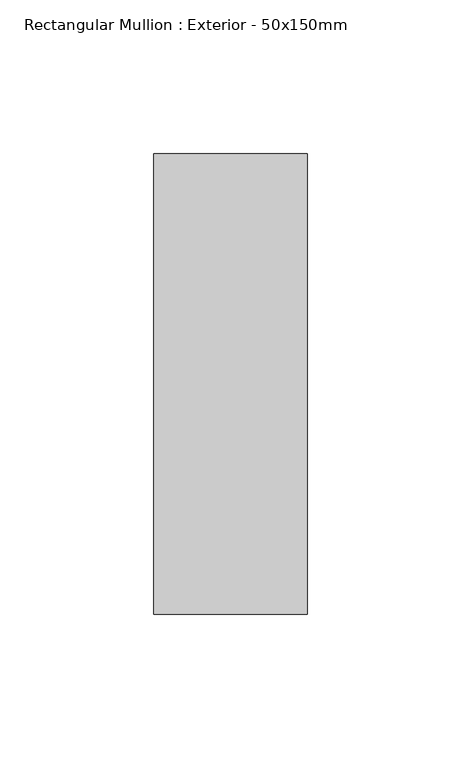
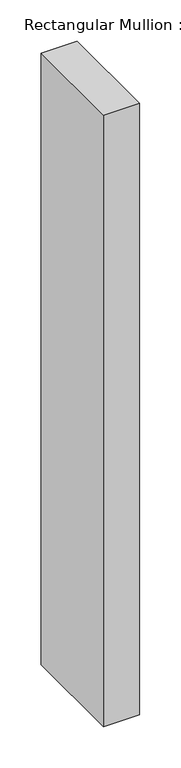
"""IFC4 building model written with IfcOpenShell, lengths in millimetres: member geometry, Rectangular Mullion : Exterior - 50x150mm."""

import ifcopenshell
import ifcopenshell.guid

model = None  # the IFC model being written
_history = None  # IfcOwnerHistory: only IFC2X3 demands one
_inside = {}  # id of a spatial element -> (the spatial element, [elements in it])
_under = {}  # id of a project, library or spatial element -> (it, [spatial elements below it])
_declared = {}  # id of a project -> (the project, [libraries it declares])
_typed = {}  # id of a type object -> (the type object, [elements of that type])
_made_of = {}  # id of a material, layer set ... -> (it, [elements and type objects made of it])


def new_model(schema):
    """Start an empty IFC model of exactly this schema.

    Asked for "IFC4X3", IfcOpenShell would pick the latest addendum, in which some entities
    have other attributes; the version numbers below select the first issue.
    IFC2X3 requires an IfcOwnerHistory on every rooted entity: one is made here for all.
    """
    global model, _history
    if schema == "IFC4X3":
        model = ifcopenshell.file(schema_version=(4, 3, 0, 0))
    else:
        model = ifcopenshell.file(schema=schema)
    _inside.clear()
    _under.clear()
    _declared.clear()
    _typed.clear()
    _made_of.clear()
    _history = None
    if model.schema == "IFC2X3":
        org = make("IfcOrganization", Name="unknown")
        user = make(
            "IfcPersonAndOrganization",
            ThePerson=make("IfcPerson", FamilyName="unknown"),
            TheOrganization=org,
        )
        app = make(
            "IfcApplication",
            ApplicationDeveloper=org,
            Version="unknown",
            ApplicationFullName="unknown",
            ApplicationIdentifier="unknown",
        )
        _history = make(
            "IfcOwnerHistory",
            OwningUser=user,
            OwningApplication=app,
            ChangeAction="ADDED",
            CreationDate=0,
        )
    return model


def make(cls, **values):
    """One entity of the class cls with the attributes given. An attribute that is None is left unset."""
    return model.create_entity(
        cls, **{name: value for name, value in values.items() if value is not None}
    )


def rooted(cls, **values):
    """An entity with a GlobalId (a new one), such as an element, a storey or a relation."""
    return make(cls, GlobalId=ifcopenshell.guid.new(), OwnerHistory=_history, **values)


def si_unit(unit_type, name, prefix=None):
    """IfcSIUnit, for example si_unit("LENGTHUNIT", "METRE", prefix="MILLI")."""
    return make("IfcSIUnit", UnitType=unit_type, Prefix=prefix, Name=name)


def assignment(units):
    """IfcUnitAssignment: the units of a project."""
    return None if units is None else make("IfcUnitAssignment", Units=units)


def point(xyz):
    """IfcCartesianPoint."""
    return None if xyz is None else make("IfcCartesianPoint", Coordinates=xyz)


def direction(xyz):
    """IfcDirection."""
    return None if xyz is None else make("IfcDirection", DirectionRatios=xyz)


def frame(location, z_axis=None, x_axis=None):
    """IfcAxis2Placement3D, a coordinate frame: its origin and axes. An axis left out is left unset."""
    return make(
        "IfcAxis2Placement3D",
        Location=point(location),
        Axis=direction(z_axis),
        RefDirection=direction(x_axis),
    )


def origin():
    """The frame at (0, 0, 0) with its axes left unset."""
    return frame((0.0, 0.0, 0.0))


def place(relative_to, where):
    """IfcLocalPlacement: puts the frame where relative to a parent placement (None: the world)."""
    return make(
        "IfcLocalPlacement", PlacementRelTo=relative_to, RelativePlacement=where
    )


def context(
    kind, dimensions, precision=None, world=None, true_north=None, identifier=None
):
    """IfcGeometricRepresentationContext, for example the 3D "Model" context."""
    return make(
        "IfcGeometricRepresentationContext",
        ContextIdentifier=identifier,
        ContextType=kind,
        CoordinateSpaceDimension=dimensions,
        Precision=precision,
        WorldCoordinateSystem=world,
        TrueNorth=true_north,
    )


def project(units=None, contexts=None):
    """IfcProject with its units and contexts."""
    return rooted(
        "IfcProject",
        Name="project",
        RepresentationContexts=contexts,
        UnitsInContext=assignment(units),
    )


def spatial(cls, under=None, at=None, **own):
    """A site, building, storey or space (cls), placed at a placement, below another one or the project."""
    s = rooted(cls, ObjectPlacement=at, **own)
    if under is not None:
        _under.setdefault(under.id(), (under, []))[1].append(s)
    return s


def polyline(points):
    """IfcPolyline through the points."""
    return make("IfcPolyline", Points=[point(p) for p in points])


def outline(outer, holes=None, kind="AREA"):
    """IfcArbitraryClosedProfileDef: a profile drawn as a closed curve; with holes, ...WithVoids."""
    if holes is None:
        return make("IfcArbitraryClosedProfileDef", ProfileType=kind, OuterCurve=outer)
    return make(
        "IfcArbitraryProfileDefWithVoids",
        ProfileType=kind,
        OuterCurve=outer,
        InnerCurves=holes,
    )


def extrude(swept, where, along, depth):
    """IfcExtrudedAreaSolid: the profile swept, set in the frame where, extruded along a direction by depth."""
    return make(
        "IfcExtrudedAreaSolid",
        SweptArea=swept,
        Position=where,
        ExtrudedDirection=direction(along),
        Depth=depth,
    )


def shape(context_of_items, identifier, shape_type, items):
    """IfcShapeRepresentation: the items that make up one representation, for example the "Body"."""
    return make(
        "IfcShapeRepresentation",
        ContextOfItems=context_of_items,
        RepresentationIdentifier=identifier,
        RepresentationType=shape_type,
        Items=items,
    )


def source(mapping_origin, context_of_items, identifier, shape_type, items):
    """IfcRepresentationMap: a shape defined once, which mapped items show again and again."""
    return make(
        "IfcRepresentationMap",
        MappingOrigin=mapping_origin,
        MappedRepresentation=shape(context_of_items, identifier, shape_type, items),
    )


def transform(
    local_origin,
    x_axis=None,
    y_axis=None,
    z_axis=None,
    scale=None,
    scale2=None,
    scale3=None,
    uniform=True,
):
    """IfcCartesianTransformationOperator3D, or its non-uniform kind. x_axis, y_axis, z_axis: its Axis1, 2, 3."""
    if uniform:
        return make(
            "IfcCartesianTransformationOperator3D",
            Axis1=direction(x_axis),
            Axis2=direction(y_axis),
            LocalOrigin=point(local_origin),
            Scale=scale,
            Axis3=direction(z_axis),
        )
    return make(
        "IfcCartesianTransformationOperator3DnonUniform",
        Axis1=direction(x_axis),
        Axis2=direction(y_axis),
        LocalOrigin=point(local_origin),
        Scale=scale,
        Axis3=direction(z_axis),
        Scale2=scale2,
        Scale3=scale3,
    )


def mapped(mapping_source, mapping_target):
    """IfcMappedItem: shows the shape of a source again, moved by a transform."""
    return make(
        "IfcMappedItem", MappingSource=mapping_source, MappingTarget=mapping_target
    )


def made_of(thing, what):
    """Note that an element or type object is made of a material, layer set ...; save() writes the relation."""
    if what is not None:
        _made_of.setdefault(what.id(), (what, []))[1].append(thing)
    return thing


def element(
    cls,
    number,
    at=None,
    inside=None,
    cuts=None,
    type_object=None,
    material=None,
    context=None,
    identifier="Body",
    shape_type=None,
    held_by="IfcProductDefinitionShape",
    body=None,
    shapes=None,
    **own,
):
    """One element of the class cls, such as IfcWall. Its Tag is "e" and its number.

    at: its placement. inside: the storey or other place that contains it. cuts: it is an
    opening in that element (IfcRelVoidsElement). A single representation is given by context,
    identifier, shape_type and body (its items); several are given by shapes. held_by: the class
    of the entity that holds the representations. save() writes the other relations.
    """
    e = rooted(cls, Tag="e%d" % number, ObjectPlacement=at, **own)
    if body is not None:
        shapes = [shape(context, identifier, shape_type, body)]
    if shapes is not None:
        e.Representation = make(held_by, Representations=shapes)
    if inside is not None:
        _inside.setdefault(inside.id(), (inside, []))[1].append(e)
    if cuts is not None:
        rooted(
            "IfcRelVoidsElement", RelatingBuildingElement=cuts, RelatedOpeningElement=e
        )
    if type_object is not None:
        _typed.setdefault(type_object.id(), (type_object, []))[1].append(e)
    return made_of(e, material)


def aggregate(whole, parts):
    """IfcRelAggregates: a whole, such as a stair, and the parts it consists of."""
    return rooted("IfcRelAggregates", RelatingObject=whole, RelatedObjects=parts)


def save(model, path):
    """Write the relations noted so far, then the file.

    IfcRelAggregates (storeys below a building ...), IfcRelContainedInSpatialStructure (elements
    in a storey), IfcRelDefinesByType, IfcRelAssociatesMaterial and IfcRelDeclares: one each for
    every whole, place, type object, material and project.
    """
    for whole, parts in _under.values():
        aggregate(whole, parts)
    for where, things in _inside.values():
        rooted(
            "IfcRelContainedInSpatialStructure",
            RelatedElements=things,
            RelatingStructure=where,
        )
    for kind, things in _typed.values():
        rooted("IfcRelDefinesByType", RelatedObjects=things, RelatingType=kind)
    for what, things in _made_of.values():
        rooted("IfcRelAssociatesMaterial", RelatedObjects=things, RelatingMaterial=what)
    for by, libraries in _declared.values():
        rooted("IfcRelDeclares", RelatingContext=by, RelatedDefinitions=libraries)
    model.write(path)


def rectangular_mullion_exterior_50x150mm_23692360(model_context):
    return source(origin(), model_context, "Body", "SweptSolid", [
        extrude(outline(polyline([(25.0, 0.0), (25.0, -150.0), (-25.0, -150.0), (-25.0, 0.0), (25.0, 0.0)])), frame((0.0, 0.0, -900.0), z_axis=(0.0, 0.0, 1.0), x_axis=(1.0, 0.0, 0.0)), (0.0, 0.0, 1.0), 900.0),
    ])


if __name__ == "__main__":
    model = new_model("IFC4")
    model_context = context("Model", 3, world=origin())
    ifc_project = project(units=[si_unit("LENGTHUNIT", "METRE", prefix="MILLI")], contexts=[model_context])
    site = spatial("IfcSite", under=ifc_project)
    building = spatial("IfcBuilding", under=site)
    placement = place(None, origin())
    rectangular_mullion_exterior_50x150mm_shape = rectangular_mullion_exterior_50x150mm_23692360(model_context)
    element("IfcMember", 1, ObjectType="Rectangular Mullion : Exterior - 50x150mm", at=placement, inside=building, context=model_context, shape_type="MappedRepresentation", body=[
        mapped(rectangular_mullion_exterior_50x150mm_shape, transform((0.0, 0.0, 0.0), x_axis=(1.0, 0.0, 0.0), y_axis=(0.0, 1.0, 0.0), z_axis=(0.0, 0.0, 1.0))),
    ])
    save(model, "model.ifc")

# Revit data of these elements
# Project information
#   Template Version = "DanEDU Building template ver. 2018.0420.0"
#   Client Name = "Test Project"
#   Project Address = "Enter address here"
#   Project Name = "3 Stories"
#   Project Number = "Number"
#   Current Version = "0.0.0"
#   SR Document GUID = "3eb9317e-835d-4f79-8926-4d15b96bc824"
# Type "Rectangular Mullion : Exterior - 50x150mm"
#   built-in parameter 1007351 = -0.246063 (stored number, unit not read)
#   built-in parameter 1007304 = 0.492126 (stored number, unit not read)
#   built-in parameter 1007301 = 0.082021 (stored number, unit not read)
#   built-in parameter 1007300 = 0.082021 (stored number, unit not read)
# Element 1 (IfcMember, "Rectangular Mullion : Exterior - 50x150mm")
#   Materials on its faces: "Default Frame/Mullion (Interior/Exterior)"
# Materials
#   "Default Frame/Mullion (Interior/Exterior)": class "Generic", colour RGB 205 205 205, transparency 0, Description = "Udefineret karm/ramme materiale", Cost = 0
